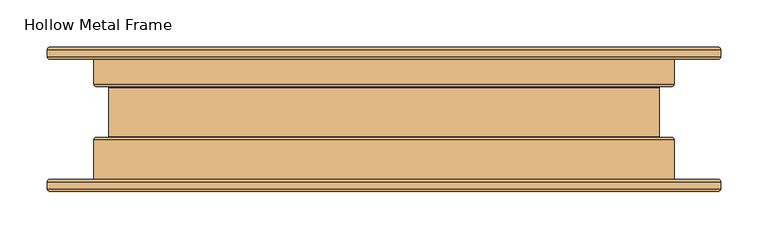
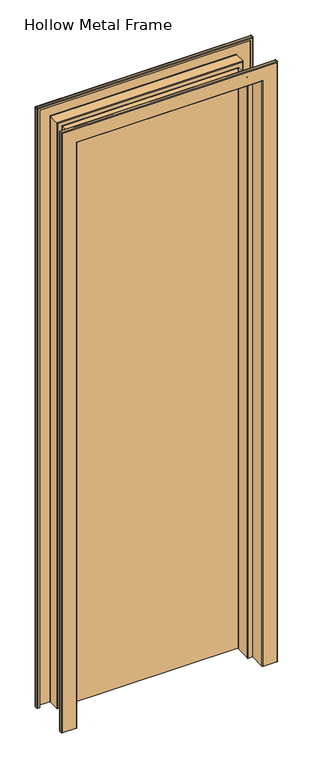
"""IFC4 building model written with IfcOpenShell, lengths in millimetres: door geometry, Hollow Metal Frame."""

from ifc_helpers import new_model, si_unit, frame, origin, origin_with_axes, place, context, project, spatial, polyline, circle_curve, ellipse_curve, outline, extrude, source, transform, mapped, element, save
from ifc_brep_helpers import plane_surface, cylinder_surface, revolved_surface, advanced_brep


def hollow_metal_frame_92897bd9(model_context):
    return source(origin(), model_context, "Body", "SolidModel", [
        advanced_brep(
        [(-353.02825, -63.5635, 0.0), (-347.6625, -63.5635, 0.0), (-347.6625, -65.11925, 0.0), (-353.02825, -65.11925, 0.0), (-354.04425, -66.13525, 0.0), (-354.04425, -73.66, 0.0), (-353.02825, -74.676, 0.0), (-307.37175, -74.676, 0.0), (-306.35575, -73.66, 0.0), (-306.35575, -21.68525, 0.0), (-303.784, -19.1135, 0.0), (-291.49675, -19.1135, 0.0), (-290.48075, -18.0975, 0.0), (-290.48075, 33.6931, 0.0), (-291.49675, 34.7091, 0.0), (-303.784, 34.7091, 0.0), (-306.35575, 37.28085, 0.0), (-306.35575, 73.5965, 0.0), (-307.37175, 74.6125, 0.0), (-353.02825, 74.6125, 0.0), (-354.04425, 73.5965, 0.0), (-354.04425, 66.07175, 0.0), (-353.02825, 65.05575, 0.0), (-347.6625, 65.05575, 0.0), (-347.6625, 63.5, 0.0), (-353.02825, 63.5, 0.0), (-355.6, 66.07175, 0.0), (-355.6, 73.5965, 0.0), (-353.02825, 76.16825, 0.0), (-307.37175, 76.16825, 0.0), (-304.8, 73.5965, 0.0), (-304.8, 37.28085, 0.0), (-303.784, 36.26485, 0.0), (-291.49675, 36.26485, 0.0), (-288.925, 33.6931, 0.0), (-288.925, -18.0975, 0.0), (-291.49675, -20.66925, 0.0), (-303.784, -20.66925, 0.0), (-304.8, -21.68525, 0.0), (-304.8, -73.66, 0.0), (-307.37175, -76.23175, 0.0), (-353.02825, -76.23175, 0.0), (-355.6, -73.66, 0.0), (-355.6, -66.13525, 0.0), (-355.6, -66.13525, 2082.8000001), (-353.02825, -63.5635, 2080.2282501), (-355.6, -73.66, 2082.8000001), (-353.02825, -76.23175, 2080.2282501), (-307.37175, -76.23175, 2034.5717501), (307.37175, -76.23175, 2034.5717501), (307.37175, -76.23175, 0.0), (353.02825, -76.23175, 0.0), (353.02825, -76.23175, 2080.2282501), (-304.8, -73.66, 2032.0000001), (-304.8, -21.68525, 2032.0000001), (-303.784, -20.66925, 2030.9840001), (-291.49675, -20.66925, 2018.6967501), (291.49675, -20.66925, 2018.6967501), (291.49675, -20.66925, 0.0), (303.784, -20.66925, 0.0), (303.784, -20.66925, 2030.9840001), (-288.925, -18.0975, 2016.1250001), (-288.925, 33.6931, 2016.1250001), (-291.49675, 36.26485, 2018.6967501), (-303.784, 36.26485, 2030.9840001), (303.784, 36.26485, 2030.9840001), (303.784, 36.26485, 0.0), (291.49675, 36.26485, 0.0), (291.49675, 36.26485, 2018.6967501), (-304.8, 37.28085, 2032.0000001), (-304.8, 73.5965, 2032.0000001), (-307.37175, 76.16825, 2034.5717501), (-353.02825, 76.16825, 2080.2282501), (353.02825, 76.16825, 2080.2282501), (353.02825, 76.16825, 0.0), (307.37175, 76.16825, 0.0), (307.37175, 76.16825, 2034.5717501), (-355.6, 73.5965, 2082.8000001), (-355.6, 66.07175, 2082.8000001), (-353.02825, 63.5, 2080.2282501), (-347.6625, 63.5, 2074.8625001), (347.6625, 63.5, 2074.8625001), (347.6625, 63.5, 0.0), (353.02825, 63.5, 0.0), (353.02825, 63.5, 2080.2282501), (-347.6625, 65.05575, 2074.8625001), (-353.02825, 65.05575, 2080.2282501), (353.02825, 65.05575, 2080.2282501), (353.02825, 65.05575, 0.0), (347.6625, 65.05575, 0.0), (347.6625, 65.05575, 2074.8625001), (-354.04425, 66.07175, 2081.2442501), (-354.04425, 73.5965, 2081.2442501), (-353.02825, 74.6125, 2080.2282501), (-307.37175, 74.6125, 2034.5717501), (307.37175, 74.6125, 2034.5717501), (307.37175, 74.6125, 0.0), (353.02825, 74.6125, 0.0), (353.02825, 74.6125, 2080.2282501), (-306.35575, 73.5965, 2033.5557501), (-306.35575, 37.28085, 2033.5557501), (-303.784, 34.7091, 2030.9840001), (-291.49675, 34.7091, 2018.6967501), (291.49675, 34.7091, 2018.6967501), (291.49675, 34.7091, 0.0), (303.784, 34.7091, 0.0), (303.784, 34.7091, 2030.9840001), (-290.48075, 33.6931, 2017.6807501), (-290.48075, -18.0975, 2017.6807501), (-291.49675, -19.1135, 2018.6967501), (-303.784, -19.1135, 2030.9840001), (303.784, -19.1135, 2030.9840001), (303.784, -19.1135, 0.0), (291.49675, -19.1135, 0.0), (291.49675, -19.1135, 2018.6967501), (-306.35575, -21.68525, 2033.5557501), (-306.35575, -73.66, 2033.5557501), (-307.37175, -74.676, 2034.5717501), (-353.02825, -74.676, 2080.2282501), (353.02825, -74.676, 2080.2282501), (353.02825, -74.676, 0.0), (307.37175, -74.676, 0.0), (307.37175, -74.676, 2034.5717501), (-354.04425, -73.66, 2081.2442501), (-354.04425, -66.13525, 2081.2442501), (-353.02825, -65.11925, 2080.2282501), (-347.6625, -65.11925, 2074.8625001), (347.6625, -65.11925, 2074.8625001), (347.6625, -65.11925, 0.0), (353.02825, -65.11925, 0.0), (353.02825, -65.11925, 2080.2282501), (-347.6625, -63.5635, 2074.8625001), (353.02825, -63.5635, 2080.2282501), (353.02825, -63.5635, 0.0), (347.6625, -63.5635, 0.0), (347.6625, -63.5635, 2074.8625001), (355.6, -66.13525, 2082.8000001), (355.6, -73.66, 2082.8000001), (304.8, -73.66, 2032.0000001), (304.8, -21.68525, 2032.0000001), (288.925, -18.0975, 2016.1250001), (288.925, 33.6931, 2016.1250001), (304.8, 37.28085, 2032.0000001), (304.8, 73.5965, 2032.0000001), (355.6, 73.5965, 2082.8000001), (355.6, 66.07175, 2082.8000001), (354.04425, 66.07175, 2081.2442501), (354.04425, 73.5965, 2081.2442501), (306.35575, 73.5965, 2033.5557501), (306.35575, 37.28085, 2033.5557501), (290.48075, 33.6931, 2017.6807501), (290.48075, -18.0975, 2017.6807501), (306.35575, -21.68525, 2033.5557501), (306.35575, -73.66, 2033.5557501), (354.04425, -73.66, 2081.2442501), (354.04425, -66.13525, 2081.2442501), (355.6, -66.13525, 0.0), (355.6, -73.66, 0.0), (304.8, -73.66, 0.0), (304.8, -21.68525, 0.0), (288.925, -18.0975, 0.0), (288.925, 33.6931, 0.0), (304.8, 37.28085, 0.0), (304.8, 73.5965, 0.0), (355.6, 73.5965, 0.0), (355.6, 66.07175, 0.0), (354.04425, 66.07175, 0.0), (354.04425, 73.5965, 0.0), (306.35575, 73.5965, 0.0), (306.35575, 37.28085, 0.0), (290.48075, 33.6931, 0.0), (290.48075, -18.0975, 0.0), (306.35575, -21.68525, 0.0), (306.35575, -73.66, 0.0), (354.04425, -73.66, 0.0), (354.04425, -66.13525, 0.0)],
        [
            (0, 1),
            (1, 2),
            (2, 3),
            (3, 4, circle_curve(frame((-353.02825, -66.13525, 0.0), z_axis=(0.0, 0.0, 1.0), x_axis=(0.0, 1.0, 0.0)), 1.016)),
            (4, 5),
            (5, 6, circle_curve(frame((-353.02825, -73.66, 0.0), z_axis=(0.0, 0.0, 1.0), x_axis=(0.0, 1.0, 0.0)), 1.016)),
            (6, 7),
            (7, 8, circle_curve(frame((-307.37175, -73.66, 0.0), z_axis=(0.0, 0.0, 1.0), x_axis=(0.0, 1.0, 0.0)), 1.016)),
            (8, 9),
            (9, 10, circle_curve(frame((-303.784, -21.68525, 0.0), z_axis=(0.0, 0.0, -1.0), x_axis=(0.0, 1.0, 0.0)), 2.57175)),
            (10, 11),
            (11, 12, circle_curve(frame((-291.49675, -18.0975, 0.0), z_axis=(0.0, 0.0, 1.0), x_axis=(0.0, 1.0, 0.0)), 1.016)),
            (12, 13),
            (13, 14, circle_curve(frame((-291.49675, 33.6931, 0.0), z_axis=(0.0, 0.0, 1.0), x_axis=(0.0, 1.0, 0.0)), 1.016)),
            (14, 15),
            (15, 16, circle_curve(frame((-303.784, 37.28085, 0.0), z_axis=(0.0, 0.0, -1.0), x_axis=(0.0, 1.0, 0.0)), 2.57175)),
            (16, 17),
            (17, 18, circle_curve(frame((-307.37175, 73.5965, 0.0), z_axis=(0.0, 0.0, 1.0), x_axis=(0.0, 1.0, 0.0)), 1.016)),
            (18, 19),
            (19, 20, circle_curve(frame((-353.02825, 73.5965, 0.0), z_axis=(0.0, 0.0, 1.0), x_axis=(0.0, 1.0, 0.0)), 1.016)),
            (20, 21),
            (21, 22, circle_curve(frame((-353.02825, 66.07175, 0.0), z_axis=(0.0, 0.0, 1.0), x_axis=(0.0, 1.0, 0.0)), 1.016)),
            (22, 23),
            (23, 24),
            (24, 25),
            (25, 26, circle_curve(frame((-353.02825, 66.07175, 0.0), z_axis=(0.0, 0.0, -1.0), x_axis=(0.0, 1.0, 0.0)), 2.57175)),
            (26, 27),
            (27, 28, circle_curve(frame((-353.02825, 73.5965, 0.0), z_axis=(0.0, 0.0, -1.0), x_axis=(0.0, 1.0, 0.0)), 2.57175)),
            (28, 29),
            (29, 30, circle_curve(frame((-307.37175, 73.5965, 0.0), z_axis=(0.0, 0.0, -1.0), x_axis=(0.0, 1.0, 0.0)), 2.57175)),
            (30, 31),
            (31, 32, circle_curve(frame((-303.784, 37.28085, 0.0), z_axis=(0.0, 0.0, 1.0), x_axis=(0.0, 1.0, 0.0)), 1.016)),
            (32, 33),
            (33, 34, circle_curve(frame((-291.49675, 33.6931, 0.0), z_axis=(0.0, 0.0, -1.0), x_axis=(0.0, 1.0, 0.0)), 2.57175)),
            (34, 35),
            (35, 36, circle_curve(frame((-291.49675, -18.0975, 0.0), z_axis=(0.0, 0.0, -1.0), x_axis=(0.0, 1.0, 0.0)), 2.57175)),
            (36, 37),
            (37, 38, circle_curve(frame((-303.784, -21.68525, 0.0), z_axis=(0.0, 0.0, 1.0), x_axis=(0.0, 1.0, 0.0)), 1.016)),
            (38, 39),
            (39, 40, circle_curve(frame((-307.37175, -73.66, 0.0), z_axis=(0.0, 0.0, -1.0), x_axis=(0.0, 1.0, 0.0)), 2.57175)),
            (40, 41),
            (41, 42, circle_curve(frame((-353.02825, -73.66, 0.0), z_axis=(0.0, 0.0, -1.0), x_axis=(0.0, 1.0, 0.0)), 2.57175)),
            (42, 43),
            (43, 0, circle_curve(frame((-353.02825, -66.13525, 0.0), z_axis=(0.0, 0.0, -1.0), x_axis=(0.0, 1.0, 0.0)), 2.57175)),
            (43, 44),
            (44, 45, ellipse_curve(frame((-353.02825, -66.13525, 2080.2282501), z_axis=(-0.7071067811865475, 0.0, -0.7071067811865475), x_axis=(0.7071067811865474, 0.0, -0.7071067811865476)), 3.6370037, 2.57175)),
            (45, 0),
            (42, 46),
            (46, 44),
            (41, 47),
            (47, 46, ellipse_curve(frame((-353.02825, -73.66, 2080.2282501), z_axis=(-0.7071067811865475, 0.0, -0.7071067811865475), x_axis=(0.7071067811865474, 0.0, -0.7071067811865476)), 3.6370037, 2.57175)),
            (40, 48),
            (48, 49),
            (49, 50),
            (50, 51),
            (51, 52),
            (52, 47),
            (39, 53),
            (53, 48, ellipse_curve(frame((-307.37175, -73.66, 2034.5717501), z_axis=(-0.7071067811865475, 0.0, -0.7071067811865475), x_axis=(0.7071067811865474, 0.0, -0.7071067811865476)), 3.6370037, 2.57175)),
            (38, 54),
            (54, 53),
            (37, 55),
            (55, 54, ellipse_curve(frame((-303.784, -21.68525, 2030.9840001), z_axis=(0.7071067811865475, 0.0, 0.7071067811865475), x_axis=(-0.7071067811865474, 0.0, 0.7071067811865476)), 1.436841, 1.016)),
            (36, 56),
            (56, 57),
            (57, 58),
            (58, 59),
            (59, 60),
            (60, 55),
            (35, 61),
            (61, 56, ellipse_curve(frame((-291.49675, -18.0975, 2018.6967501), z_axis=(-0.7071067811865475, 0.0, -0.7071067811865475), x_axis=(0.7071067811865474, 0.0, -0.7071067811865476)), 3.6370037, 2.57175)),
            (34, 62),
            (62, 61),
            (33, 63),
            (63, 62, ellipse_curve(frame((-291.49675, 33.6931, 2018.6967501), z_axis=(-0.7071067811865475, 0.0, -0.7071067811865475), x_axis=(0.7071067811865474, 0.0, -0.7071067811865476)), 3.6370037, 2.57175)),
            (32, 64),
            (64, 65),
            (65, 66),
            (66, 67),
            (67, 68),
            (68, 63),
            (31, 69),
            (69, 64, ellipse_curve(frame((-303.784, 37.28085, 2030.9840001), z_axis=(0.7071067811865475, 0.0, 0.7071067811865475), x_axis=(-0.7071067811865474, 0.0, 0.7071067811865476)), 1.436841, 1.016)),
            (30, 70),
            (70, 69),
            (29, 71),
            (71, 70, ellipse_curve(frame((-307.37175, 73.5965, 2034.5717501), z_axis=(-0.7071067811865475, 0.0, -0.7071067811865475), x_axis=(0.7071067811865474, 0.0, -0.7071067811865476)), 3.6370037, 2.57175)),
            (28, 72),
            (72, 73),
            (73, 74),
            (74, 75),
            (75, 76),
            (76, 71),
            (27, 77),
            (77, 72, ellipse_curve(frame((-353.02825, 73.5965, 2080.2282501), z_axis=(-0.7071067811865475, 0.0, -0.7071067811865475), x_axis=(0.7071067811865474, 0.0, -0.7071067811865476)), 3.6370037, 2.57175)),
            (26, 78),
            (78, 77),
            (25, 79),
            (79, 78, ellipse_curve(frame((-353.02825, 66.07175, 2080.2282501), z_axis=(-0.7071067811865475, 0.0, -0.7071067811865475), x_axis=(0.7071067811865474, 0.0, -0.7071067811865476)), 3.6370037, 2.57175)),
            (24, 80),
            (80, 81),
            (81, 82),
            (82, 83),
            (83, 84),
            (84, 79),
            (23, 85),
            (85, 80),
            (22, 86),
            (86, 87),
            (87, 88),
            (88, 89),
            (89, 90),
            (90, 85),
            (21, 91),
            (91, 86, ellipse_curve(frame((-353.02825, 66.07175, 2080.2282501), z_axis=(0.7071067811865475, 0.0, 0.7071067811865475), x_axis=(-0.7071067811865474, 0.0, 0.7071067811865476)), 1.436841, 1.016)),
            (20, 92),
            (92, 91),
            (19, 93),
            (93, 92, ellipse_curve(frame((-353.02825, 73.5965, 2080.2282501), z_axis=(0.7071067811865475, 0.0, 0.7071067811865475), x_axis=(-0.7071067811865474, 0.0, 0.7071067811865476)), 1.436841, 1.016)),
            (18, 94),
            (94, 95),
            (95, 96),
            (96, 97),
            (97, 98),
            (98, 93),
            (17, 99),
            (99, 94, ellipse_curve(frame((-307.37175, 73.5965, 2034.5717501), z_axis=(0.7071067811865475, 0.0, 0.7071067811865475), x_axis=(-0.7071067811865474, 0.0, 0.7071067811865476)), 1.436841, 1.016)),
            (16, 100),
            (100, 99),
            (15, 101),
            (101, 100, ellipse_curve(frame((-303.784, 37.28085, 2030.9840001), z_axis=(-0.7071067811865475, 0.0, -0.7071067811865475), x_axis=(0.7071067811865474, 0.0, -0.7071067811865476)), 3.6370037, 2.57175)),
            (14, 102),
            (102, 103),
            (103, 104),
            (104, 105),
            (105, 106),
            (106, 101),
            (13, 107),
            (107, 102, ellipse_curve(frame((-291.49675, 33.6931, 2018.6967501), z_axis=(0.7071067811865475, 0.0, 0.7071067811865475), x_axis=(-0.7071067811865474, 0.0, 0.7071067811865476)), 1.436841, 1.016)),
            (12, 108),
            (108, 107),
            (11, 109),
            (109, 108, ellipse_curve(frame((-291.49675, -18.0975, 2018.6967501), z_axis=(0.7071067811865475, 0.0, 0.7071067811865475), x_axis=(-0.7071067811865474, 0.0, 0.7071067811865476)), 1.436841, 1.016)),
            (10, 110),
            (110, 111),
            (111, 112),
            (112, 113),
            (113, 114),
            (114, 109),
            (9, 115),
            (115, 110, ellipse_curve(frame((-303.784, -21.68525, 2030.9840001), z_axis=(-0.7071067811865475, 0.0, -0.7071067811865475), x_axis=(0.7071067811865474, 0.0, -0.7071067811865476)), 3.6370037, 2.57175)),
            (8, 116),
            (116, 115),
            (7, 117),
            (117, 116, ellipse_curve(frame((-307.37175, -73.66, 2034.5717501), z_axis=(0.7071067811865475, 0.0, 0.7071067811865475), x_axis=(-0.7071067811865474, 0.0, 0.7071067811865476)), 1.436841, 1.016)),
            (6, 118),
            (118, 119),
            (119, 120),
            (120, 121),
            (121, 122),
            (122, 117),
            (5, 123),
            (123, 118, ellipse_curve(frame((-353.02825, -73.66, 2080.2282501), z_axis=(0.7071067811865475, 0.0, 0.7071067811865475), x_axis=(-0.7071067811865474, 0.0, 0.7071067811865476)), 1.436841, 1.016)),
            (4, 124),
            (124, 123),
            (3, 125),
            (125, 124, ellipse_curve(frame((-353.02825, -66.13525, 2080.2282501), z_axis=(0.7071067811865475, 0.0, 0.7071067811865475), x_axis=(-0.7071067811865474, 0.0, 0.7071067811865476)), 1.436841, 1.016)),
            (2, 126),
            (126, 127),
            (127, 128),
            (128, 129),
            (129, 130),
            (130, 125),
            (1, 131),
            (131, 126),
            (45, 132),
            (132, 133),
            (133, 134),
            (134, 135),
            (135, 131),
            (44, 136),
            (136, 132, ellipse_curve(frame((353.02825, -66.13525, 2080.2282501), z_axis=(-0.7071067811865475, 0.0, 0.7071067811865475), x_axis=(-0.7071067811865476, 0.0, -0.7071067811865474)), 3.6370037, 2.57175)),
            (46, 137),
            (137, 136),
            (52, 137, ellipse_curve(frame((353.02825, -73.66, 2080.2282501), z_axis=(-0.7071067811865475, 0.0, 0.7071067811865475), x_axis=(-0.7071067811865476, 0.0, -0.7071067811865474)), 3.6370037, 2.57175)),
            (53, 138),
            (138, 49, ellipse_curve(frame((307.37175, -73.66, 2034.5717501), z_axis=(-0.7071067811865475, 0.0, 0.7071067811865475), x_axis=(-0.7071067811865476, 0.0, -0.7071067811865474)), 3.6370037, 2.57175)),
            (54, 139),
            (139, 138),
            (60, 139, ellipse_curve(frame((303.784, -21.68525, 2030.9840001), z_axis=(0.7071067811865475, 0.0, -0.7071067811865475), x_axis=(0.7071067811865476, 0.0, 0.7071067811865474)), 1.436841, 1.016)),
            (61, 140),
            (140, 57, ellipse_curve(frame((291.49675, -18.0975, 2018.6967501), z_axis=(-0.7071067811865475, 0.0, 0.7071067811865475), x_axis=(-0.7071067811865476, 0.0, -0.7071067811865474)), 3.6370037, 2.57175)),
            (62, 141),
            (141, 140),
            (68, 141, ellipse_curve(frame((291.49675, 33.6931, 2018.6967501), z_axis=(-0.7071067811865475, 0.0, 0.7071067811865475), x_axis=(-0.7071067811865476, 0.0, -0.7071067811865474)), 3.6370037, 2.57175)),
            (69, 142),
            (142, 65, ellipse_curve(frame((303.784, 37.28085, 2030.9840001), z_axis=(0.7071067811865475, 0.0, -0.7071067811865475), x_axis=(0.7071067811865476, 0.0, 0.7071067811865474)), 1.436841, 1.016)),
            (70, 143),
            (143, 142),
            (76, 143, ellipse_curve(frame((307.37175, 73.5965, 2034.5717501), z_axis=(-0.7071067811865475, 0.0, 0.7071067811865475), x_axis=(-0.7071067811865476, 0.0, -0.7071067811865474)), 3.6370037, 2.57175)),
            (77, 144),
            (144, 73, ellipse_curve(frame((353.02825, 73.5965, 2080.2282501), z_axis=(-0.7071067811865475, 0.0, 0.7071067811865475), x_axis=(-0.7071067811865476, 0.0, -0.7071067811865474)), 3.6370037, 2.57175)),
            (78, 145),
            (145, 144),
            (84, 145, ellipse_curve(frame((353.02825, 66.07175, 2080.2282501), z_axis=(-0.7071067811865475, 0.0, 0.7071067811865475), x_axis=(-0.7071067811865476, 0.0, -0.7071067811865474)), 3.6370037, 2.57175)),
            (90, 81),
            (91, 146),
            (146, 87, ellipse_curve(frame((353.02825, 66.07175, 2080.2282501), z_axis=(0.7071067811865475, 0.0, -0.7071067811865475), x_axis=(0.7071067811865476, 0.0, 0.7071067811865474)), 1.436841, 1.016)),
            (92, 147),
            (147, 146),
            (98, 147, ellipse_curve(frame((353.02825, 73.5965, 2080.2282501), z_axis=(0.7071067811865475, 0.0, -0.7071067811865475), x_axis=(0.7071067811865476, 0.0, 0.7071067811865474)), 1.436841, 1.016)),
            (99, 148),
            (148, 95, ellipse_curve(frame((307.37175, 73.5965, 2034.5717501), z_axis=(0.7071067811865475, 0.0, -0.7071067811865475), x_axis=(0.7071067811865476, 0.0, 0.7071067811865474)), 1.436841, 1.016)),
            (100, 149),
            (149, 148),
            (106, 149, ellipse_curve(frame((303.784, 37.28085, 2030.9840001), z_axis=(-0.7071067811865475, 0.0, 0.7071067811865475), x_axis=(-0.7071067811865476, 0.0, -0.7071067811865474)), 3.6370037, 2.57175)),
            (107, 150),
            (150, 103, ellipse_curve(frame((291.49675, 33.6931, 2018.6967501), z_axis=(0.7071067811865475, 0.0, -0.7071067811865475), x_axis=(0.7071067811865476, 0.0, 0.7071067811865474)), 1.436841, 1.016)),
            (108, 151),
            (151, 150),
            (114, 151, ellipse_curve(frame((291.49675, -18.0975, 2018.6967501), z_axis=(0.7071067811865475, 0.0, -0.7071067811865475), x_axis=(0.7071067811865476, 0.0, 0.7071067811865474)), 1.436841, 1.016)),
            (115, 152),
            (152, 111, ellipse_curve(frame((303.784, -21.68525, 2030.9840001), z_axis=(-0.7071067811865475, 0.0, 0.7071067811865475), x_axis=(-0.7071067811865476, 0.0, -0.7071067811865474)), 3.6370037, 2.57175)),
            (116, 153),
            (153, 152),
            (122, 153, ellipse_curve(frame((307.37175, -73.66, 2034.5717501), z_axis=(0.7071067811865475, 0.0, -0.7071067811865475), x_axis=(0.7071067811865476, 0.0, 0.7071067811865474)), 1.436841, 1.016)),
            (123, 154),
            (154, 119, ellipse_curve(frame((353.02825, -73.66, 2080.2282501), z_axis=(0.7071067811865475, 0.0, -0.7071067811865475), x_axis=(0.7071067811865476, 0.0, 0.7071067811865474)), 1.436841, 1.016)),
            (124, 155),
            (155, 154),
            (130, 155, ellipse_curve(frame((353.02825, -66.13525, 2080.2282501), z_axis=(0.7071067811865475, 0.0, -0.7071067811865475), x_axis=(0.7071067811865476, 0.0, 0.7071067811865474)), 1.436841, 1.016)),
            (135, 127),
            (133, 156, circle_curve(frame((353.02825, -66.13525, 0.0), z_axis=(0.0, 0.0, -1.0), x_axis=(0.0, 1.0, 0.0)), 2.57175)),
            (156, 157),
            (157, 51, circle_curve(frame((353.02825, -73.66, 0.0), z_axis=(0.0, 0.0, -1.0), x_axis=(0.0, 1.0, 0.0)), 2.57175)),
            (50, 158, circle_curve(frame((307.37175, -73.66, 0.0), z_axis=(0.0, 0.0, -1.0), x_axis=(0.0, 1.0, 0.0)), 2.57175)),
            (158, 159),
            (159, 59, circle_curve(frame((303.784, -21.68525, 0.0), z_axis=(0.0, 0.0, 1.0), x_axis=(0.0, 1.0, 0.0)), 1.016)),
            (58, 160, circle_curve(frame((291.49675, -18.0975, 0.0), z_axis=(0.0, 0.0, -1.0), x_axis=(0.0, 1.0, 0.0)), 2.57175)),
            (160, 161),
            (161, 67, circle_curve(frame((291.49675, 33.6931, 0.0), z_axis=(0.0, 0.0, -1.0), x_axis=(0.0, 1.0, 0.0)), 2.57175)),
            (66, 162, circle_curve(frame((303.784, 37.28085, 0.0), z_axis=(0.0, 0.0, 1.0), x_axis=(0.0, 1.0, 0.0)), 1.016)),
            (162, 163),
            (163, 75, circle_curve(frame((307.37175, 73.5965, 0.0), z_axis=(0.0, 0.0, -1.0), x_axis=(0.0, 1.0, 0.0)), 2.57175)),
            (74, 164, circle_curve(frame((353.02825, 73.5965, 0.0), z_axis=(0.0, 0.0, -1.0), x_axis=(0.0, 1.0, 0.0)), 2.57175)),
            (164, 165),
            (165, 83, circle_curve(frame((353.02825, 66.07175, 0.0), z_axis=(0.0, 0.0, -1.0), x_axis=(0.0, 1.0, 0.0)), 2.57175)),
            (82, 89),
            (88, 166, circle_curve(frame((353.02825, 66.07175, 0.0), z_axis=(0.0, 0.0, 1.0), x_axis=(0.0, 1.0, 0.0)), 1.016)),
            (166, 167),
            (167, 97, circle_curve(frame((353.02825, 73.5965, 0.0), z_axis=(0.0, 0.0, 1.0), x_axis=(0.0, 1.0, 0.0)), 1.016)),
            (96, 168, circle_curve(frame((307.37175, 73.5965, 0.0), z_axis=(0.0, 0.0, 1.0), x_axis=(0.0, 1.0, 0.0)), 1.016)),
            (168, 169),
            (169, 105, circle_curve(frame((303.784, 37.28085, 0.0), z_axis=(0.0, 0.0, -1.0), x_axis=(0.0, 1.0, 0.0)), 2.57175)),
            (104, 170, circle_curve(frame((291.49675, 33.6931, 0.0), z_axis=(0.0, 0.0, 1.0), x_axis=(0.0, 1.0, 0.0)), 1.016)),
            (170, 171),
            (171, 113, circle_curve(frame((291.49675, -18.0975, 0.0), z_axis=(0.0, 0.0, 1.0), x_axis=(0.0, 1.0, 0.0)), 1.016)),
            (112, 172, circle_curve(frame((303.784, -21.68525, 0.0), z_axis=(0.0, 0.0, -1.0), x_axis=(0.0, 1.0, 0.0)), 2.57175)),
            (172, 173),
            (173, 121, circle_curve(frame((307.37175, -73.66, 0.0), z_axis=(0.0, 0.0, 1.0), x_axis=(0.0, 1.0, 0.0)), 1.016)),
            (120, 174, circle_curve(frame((353.02825, -73.66, 0.0), z_axis=(0.0, 0.0, 1.0), x_axis=(0.0, 1.0, 0.0)), 1.016)),
            (174, 175),
            (175, 129, circle_curve(frame((353.02825, -66.13525, 0.0), z_axis=(0.0, 0.0, 1.0), x_axis=(0.0, 1.0, 0.0)), 1.016)),
            (128, 134),
            (136, 156),
            (137, 157),
            (138, 158),
            (139, 159),
            (140, 160),
            (141, 161),
            (142, 162),
            (143, 163),
            (144, 164),
            (145, 165),
            (146, 166),
            (147, 167),
            (148, 168),
            (149, 169),
            (150, 170),
            (151, 171),
            (152, 172),
            (153, 173),
            (154, 174),
            (155, 175),
        ],
        [
            plane_surface(frame((-315.9125, 63.5, 0.0), z_axis=(0.0, 0.0, -1.0), x_axis=(1.0, 0.0, 0.0))),
            cylinder_surface(frame((-353.02825, -66.13525, 0.0), z_axis=(0.0, 0.0, -1.0), x_axis=(0.0, 1.0, 0.0)), 2.57175),
            plane_surface(frame((-355.6, -66.13525, 0.0), z_axis=(-1.0, 0.0, 0.0), x_axis=(0.0, 0.0, 1.0))),
            cylinder_surface(frame((-353.02825, -73.66, 0.0), z_axis=(0.0, 0.0, -1.0), x_axis=(0.0, 1.0, 0.0)), 2.57175),
            plane_surface(frame((-353.02825, -76.23175, 0.0), z_axis=(0.0, -1.0, 0.0), x_axis=(0.0, 0.0, 1.0))),
            cylinder_surface(frame((-307.37175, -73.66, 0.0), z_axis=(0.0, 0.0, -1.0), x_axis=(0.0, 1.0, 0.0)), 2.57175),
            plane_surface(frame((-304.8, -73.66, 0.0), z_axis=(1.0, 0.0, 0.0), x_axis=(0.0, 0.0, 1.0))),
            revolved_surface(polyline([(-303.784, -20.669249999999998, 2032.0000001145868), (-303.784, -20.669249999999998, 0.0)]), (-303.784, -21.68525, 0.0), (0.0, 0.0, 1.0)),
            plane_surface(frame((-303.784, -20.66925, 0.0), z_axis=(0.0, -1.0, 0.0), x_axis=(0.0, 0.0, 1.0))),
            cylinder_surface(frame((-291.49675, -18.0975, 0.0), z_axis=(0.0, 0.0, -1.0), x_axis=(0.0, 1.0, 0.0)), 2.57175),
            plane_surface(frame((-288.925, -18.0975, 0.0), z_axis=(1.0, 0.0, 0.0), x_axis=(0.0, 0.0, 1.0))),
            cylinder_surface(frame((-291.49675, 33.6931, 0.0), z_axis=(0.0, 0.0, -1.0), x_axis=(0.0, 1.0, 0.0)), 2.57175),
            plane_surface(frame((-291.49675, 36.26485, 0.0), z_axis=(0.0, 1.0, 0.0), x_axis=(0.0, 0.0, 1.0))),
            revolved_surface(polyline([(-303.784, 38.29685, 2032.0000001145868), (-303.784, 38.29685, 0.0)]), (-303.784, 37.28085, 0.0), (0.0, 0.0, 1.0)),
            plane_surface(frame((-304.8, 37.28085, 0.0), z_axis=(1.0, 0.0, 0.0), x_axis=(0.0, 0.0, 1.0))),
            cylinder_surface(frame((-307.37175, 73.5965, 0.0), z_axis=(0.0, 0.0, -1.0), x_axis=(0.0, 1.0, 0.0)), 2.57175),
            plane_surface(frame((-307.37175, 76.16825, 0.0), z_axis=(0.0, 1.0, 0.0), x_axis=(0.0, 0.0, 1.0))),
            cylinder_surface(frame((-353.02825, 73.5965, 0.0), z_axis=(0.0, 0.0, -1.0), x_axis=(0.0, 1.0, 0.0)), 2.57175),
            plane_surface(frame((-355.6, 73.5965, 0.0), z_axis=(-1.0, 0.0, 0.0), x_axis=(0.0, 0.0, 1.0))),
            cylinder_surface(frame((-353.02825, 66.07175, 0.0), z_axis=(0.0, 0.0, -1.0), x_axis=(0.0, 1.0, 0.0)), 2.57175),
            plane_surface(frame((-353.02825, 63.5, 0.0), z_axis=(0.0, -1.0, 0.0), x_axis=(0.0, 0.0, 1.0))),
            plane_surface(frame((-347.6625, 63.5, 0.0), z_axis=(1.0, 0.0, 0.0), x_axis=(0.0, 0.0, 1.0))),
            plane_surface(frame((-347.6625, 65.05575, 0.0), z_axis=(0.0, 1.0, 0.0), x_axis=(0.0, 0.0, 1.0))),
            revolved_surface(polyline([(-353.02825, 67.08775, 2081.244250114587), (-353.02825, 67.08775, 0.0)]), (-353.02825, 66.07175, 0.0), (0.0, 0.0, 1.0)),
            plane_surface(frame((-354.04425, 66.07175, 0.0), z_axis=(1.0, 0.0, 0.0), x_axis=(0.0, 0.0, 1.0))),
            revolved_surface(polyline([(-353.02825, 74.61250000000001, 2081.244250114587), (-353.02825, 74.61250000000001, 0.0)]), (-353.02825, 73.5965, 0.0), (0.0, 0.0, 1.0)),
            plane_surface(frame((-353.02825, 74.6125, 0.0), z_axis=(0.0, -1.0, 0.0), x_axis=(0.0, 0.0, 1.0))),
            revolved_surface(polyline([(-307.37175, 74.61250000000001, 2035.5877501145867), (-307.37175, 74.61250000000001, 0.0)]), (-307.37175, 73.5965, 0.0), (0.0, 0.0, 1.0)),
            plane_surface(frame((-306.35575, 73.5965, 0.0), z_axis=(-1.0, 0.0, 0.0), x_axis=(0.0, 0.0, 1.0))),
            cylinder_surface(frame((-303.784, 37.28085, 0.0), z_axis=(0.0, 0.0, -1.0), x_axis=(0.0, 1.0, 0.0)), 2.57175),
            plane_surface(frame((-303.784, 34.7091, 0.0), z_axis=(0.0, -1.0, 0.0), x_axis=(0.0, 0.0, 1.0))),
            revolved_surface(polyline([(-291.49675, 34.7091, 2019.7127501145867), (-291.49675, 34.7091, 0.0)]), (-291.49675, 33.6931, 0.0), (0.0, 0.0, 1.0)),
            plane_surface(frame((-290.48075, 33.6931, 0.0), z_axis=(-1.0, 0.0, 0.0), x_axis=(0.0, 0.0, 1.0))),
            revolved_surface(polyline([(-291.49675, -17.0815, 2019.7127501145867), (-291.49675, -17.0815, 0.0)]), (-291.49675, -18.0975, 0.0), (0.0, 0.0, 1.0)),
            plane_surface(frame((-291.49675, -19.1135, 0.0), z_axis=(0.0, 1.0, 0.0), x_axis=(0.0, 0.0, 1.0))),
            cylinder_surface(frame((-303.784, -21.68525, 0.0), z_axis=(0.0, 0.0, -1.0), x_axis=(0.0, 1.0, 0.0)), 2.57175),
            plane_surface(frame((-306.35575, -21.68525, 0.0), z_axis=(-1.0, 0.0, 0.0), x_axis=(0.0, 0.0, 1.0))),
            revolved_surface(polyline([(-307.37175, -72.64399999999999, 2035.5877501145867), (-307.37175, -72.64399999999999, 0.0)]), (-307.37175, -73.66, 0.0), (0.0, 0.0, 1.0)),
            plane_surface(frame((-307.37175, -74.676, 0.0), z_axis=(0.0, 1.0, 0.0), x_axis=(0.0, 0.0, 1.0))),
            revolved_surface(polyline([(-353.02825, -72.64399999999999, 2081.244250114587), (-353.02825, -72.64399999999999, 0.0)]), (-353.02825, -73.66, 0.0), (0.0, 0.0, 1.0)),
            plane_surface(frame((-354.04425, -73.66, 0.0), z_axis=(1.0, 0.0, 0.0), x_axis=(0.0, 0.0, 1.0))),
            revolved_surface(polyline([(-353.02825, -65.11925, 2081.244250114587), (-353.02825, -65.11925, 0.0)]), (-353.02825, -66.13525, 0.0), (0.0, 0.0, 1.0)),
            plane_surface(frame((-353.02825, -65.11925, 0.0), z_axis=(0.0, -1.0, 0.0), x_axis=(0.0, 0.0, 1.0))),
            plane_surface(frame((-347.6625, -65.11925, 0.0), z_axis=(1.0, 0.0, 0.0), x_axis=(0.0, 0.0, 1.0))),
            plane_surface(frame((-347.6625, -63.5635, 0.0), z_axis=(0.0, 1.0, 0.0), x_axis=(0.0, 0.0, 1.0))),
            cylinder_surface(frame((-315.9125, -66.13525, 2080.2282501), z_axis=(-1.0, 0.0, 0.0), x_axis=(0.0, 1.0, 0.0)), 2.57175),
            plane_surface(frame((-355.6, -66.13525, 2082.8000001), z_axis=(0.0, 0.0, 1.0), x_axis=(1.0, 0.0, 0.0))),
            cylinder_surface(frame((-315.9125, -73.66, 2080.2282501), z_axis=(-1.0, 0.0, 0.0), x_axis=(0.0, 1.0, 0.0)), 2.57175),
            cylinder_surface(frame((-315.9125, -73.66, 2034.5717501), z_axis=(-1.0, 0.0, 0.0), x_axis=(0.0, 1.0, 0.0)), 2.57175),
            plane_surface(frame((-304.8, -73.66, 2032.0000001), z_axis=(0.0, 0.0, -1.0), x_axis=(1.0, 0.0, 0.0))),
            revolved_surface(polyline([(304.8000000145869, -20.669249999999998, 2030.9840001), (-304.80000001458683, -20.669249999999998, 2030.9840001)]), (-315.9125, -21.68525, 2030.9840001), (1.0, 0.0, 0.0)),
            cylinder_surface(frame((-315.9125, -18.0975, 2018.6967501), z_axis=(-1.0, 0.0, 0.0), x_axis=(0.0, 1.0, 0.0)), 2.57175),
            plane_surface(frame((-288.925, -18.0975, 2016.1250001), z_axis=(0.0, 0.0, -1.0), x_axis=(1.0, 0.0, 0.0))),
            cylinder_surface(frame((-315.9125, 33.6931, 2018.6967501), z_axis=(-1.0, 0.0, 0.0), x_axis=(0.0, 1.0, 0.0)), 2.57175),
            revolved_surface(polyline([(304.8000000145869, 38.29685, 2030.9840001), (-304.80000001458683, 38.29685, 2030.9840001)]), (-315.9125, 37.28085, 2030.9840001), (1.0, 0.0, 0.0)),
            plane_surface(frame((-304.8, 37.28085, 2032.0000001), z_axis=(0.0, 0.0, -1.0), x_axis=(1.0, 0.0, 0.0))),
            cylinder_surface(frame((-315.9125, 73.5965, 2034.5717501), z_axis=(-1.0, 0.0, 0.0), x_axis=(0.0, 1.0, 0.0)), 2.57175),
            cylinder_surface(frame((-315.9125, 73.5965, 2080.2282501), z_axis=(-1.0, 0.0, 0.0), x_axis=(0.0, 1.0, 0.0)), 2.57175),
            plane_surface(frame((-355.6, 73.5965, 2082.8000001), z_axis=(0.0, 0.0, 1.0), x_axis=(1.0, 0.0, 0.0))),
            cylinder_surface(frame((-315.9125, 66.07175, 2080.2282501), z_axis=(-1.0, 0.0, 0.0), x_axis=(0.0, 1.0, 0.0)), 2.57175),
            plane_surface(frame((-347.6625, 63.5, 2074.8625001), z_axis=(0.0, 0.0, -1.0), x_axis=(1.0, 0.0, 0.0))),
            revolved_surface(polyline([(354.04425001458685, 67.08775, 2080.2282501), (-354.04425001458685, 67.08775, 2080.2282501)]), (-315.9125, 66.07175, 2080.2282501), (1.0, 0.0, 0.0)),
            plane_surface(frame((-354.04425, 66.07175, 2081.2442501), z_axis=(0.0, 0.0, -1.0), x_axis=(1.0, 0.0, 0.0))),
            revolved_surface(polyline([(354.04425001458685, 74.61250000000001, 2080.2282501), (-354.04425001458685, 74.61250000000001, 2080.2282501)]), (-315.9125, 73.5965, 2080.2282501), (1.0, 0.0, 0.0)),
            revolved_surface(polyline([(308.3877500145869, 74.61250000000001, 2034.5717501), (-308.38775001458686, 74.61250000000001, 2034.5717501)]), (-315.9125, 73.5965, 2034.5717501), (1.0, 0.0, 0.0)),
            plane_surface(frame((-306.35575, 73.5965, 2033.5557501), z_axis=(0.0, 0.0, 1.0), x_axis=(1.0, 0.0, 0.0))),
            cylinder_surface(frame((-315.9125, 37.28085, 2030.9840001), z_axis=(-1.0, 0.0, 0.0), x_axis=(0.0, 1.0, 0.0)), 2.57175),
            revolved_surface(polyline([(292.5127500145869, 34.7091, 2018.6967501), (-292.51275001458686, 34.7091, 2018.6967501)]), (-315.9125, 33.6931, 2018.6967501), (1.0, 0.0, 0.0)),
            plane_surface(frame((-290.48075, 33.6931, 2017.6807501), z_axis=(0.0, 0.0, 1.0), x_axis=(1.0, 0.0, 0.0))),
            revolved_surface(polyline([(292.5127500145869, -17.0815, 2018.6967501), (-292.51275001458686, -17.0815, 2018.6967501)]), (-315.9125, -18.0975, 2018.6967501), (1.0, 0.0, 0.0)),
            cylinder_surface(frame((-315.9125, -21.68525, 2030.9840001), z_axis=(-1.0, 0.0, 0.0), x_axis=(0.0, 1.0, 0.0)), 2.57175),
            plane_surface(frame((-306.35575, -21.68525, 2033.5557501), z_axis=(0.0, 0.0, 1.0), x_axis=(1.0, 0.0, 0.0))),
            revolved_surface(polyline([(308.3877500145869, -72.64399999999999, 2034.5717501), (-308.38775001458686, -72.64399999999999, 2034.5717501)]), (-315.9125, -73.66, 2034.5717501), (1.0, 0.0, 0.0)),
            revolved_surface(polyline([(354.04425001458685, -72.64399999999999, 2080.2282501), (-354.04425001458685, -72.64399999999999, 2080.2282501)]), (-315.9125, -73.66, 2080.2282501), (1.0, 0.0, 0.0)),
            plane_surface(frame((-354.04425, -73.66, 2081.2442501), z_axis=(0.0, 0.0, -1.0), x_axis=(1.0, 0.0, 0.0))),
            revolved_surface(polyline([(354.04425001458685, -65.11925, 2080.2282501), (-354.04425001458685, -65.11925, 2080.2282501)]), (-315.9125, -66.13525, 2080.2282501), (1.0, 0.0, 0.0)),
            plane_surface(frame((-347.6625, -65.11925, 2074.8625001), z_axis=(0.0, 0.0, -1.0), x_axis=(1.0, 0.0, 0.0))),
            plane_surface(frame((315.9125, 63.5, 0.0), z_axis=(0.0, 0.0, -1.0), x_axis=(-1.0, 0.0, 0.0))),
            cylinder_surface(frame((353.02825, -66.13525, 2043.1125001), z_axis=(0.0, 0.0, 1.0), x_axis=(0.0, 1.0, 0.0)), 2.57175),
            plane_surface(frame((355.6, -66.13525, 2082.8000001), z_axis=(1.0, 0.0, 0.0), x_axis=(0.0, 0.0, -1.0))),
            cylinder_surface(frame((353.02825, -73.66, 2043.1125001), z_axis=(0.0, 0.0, 1.0), x_axis=(0.0, 1.0, 0.0)), 2.57175),
            cylinder_surface(frame((307.37175, -73.66, 2043.1125001), z_axis=(0.0, 0.0, 1.0), x_axis=(0.0, 1.0, 0.0)), 2.57175),
            plane_surface(frame((304.8, -73.66, 2032.0000001), z_axis=(-1.0, 0.0, 0.0), x_axis=(0.0, 0.0, -1.0))),
            revolved_surface(polyline([(303.784, -20.669249999999998, 0.0), (303.784, -20.669249999999998, 2032.0000001145868)]), (303.784, -21.68525, 2043.1125001), (0.0, 0.0, -1.0)),
            cylinder_surface(frame((291.49675, -18.0975, 2043.1125001), z_axis=(0.0, 0.0, 1.0), x_axis=(0.0, 1.0, 0.0)), 2.57175),
            plane_surface(frame((288.925, -18.0975, 2016.1250001), z_axis=(-1.0, 0.0, 0.0), x_axis=(0.0, 0.0, -1.0))),
            cylinder_surface(frame((291.49675, 33.6931, 2043.1125001), z_axis=(0.0, 0.0, 1.0), x_axis=(0.0, 1.0, 0.0)), 2.57175),
            revolved_surface(polyline([(303.784, 38.29685, 0.0), (303.784, 38.29685, 2032.0000001145868)]), (303.784, 37.28085, 2043.1125001), (0.0, 0.0, -1.0)),
            plane_surface(frame((304.8, 37.28085, 2032.0000001), z_axis=(-1.0, 0.0, 0.0), x_axis=(0.0, 0.0, -1.0))),
            cylinder_surface(frame((307.37175, 73.5965, 2043.1125001), z_axis=(0.0, 0.0, 1.0), x_axis=(0.0, 1.0, 0.0)), 2.57175),
            cylinder_surface(frame((353.02825, 73.5965, 2043.1125001), z_axis=(0.0, 0.0, 1.0), x_axis=(0.0, 1.0, 0.0)), 2.57175),
            plane_surface(frame((355.6, 73.5965, 2082.8000001), z_axis=(1.0, 0.0, 0.0), x_axis=(0.0, 0.0, -1.0))),
            cylinder_surface(frame((353.02825, 66.07175, 2043.1125001), z_axis=(0.0, 0.0, 1.0), x_axis=(0.0, 1.0, 0.0)), 2.57175),
            plane_surface(frame((347.6625, 63.5, 2074.8625001), z_axis=(-1.0, 0.0, 0.0), x_axis=(0.0, 0.0, -1.0))),
            revolved_surface(polyline([(353.02825, 67.08775, 0.0), (353.02825, 67.08775, 2081.244250114587)]), (353.02825, 66.07175, 2043.1125001), (0.0, 0.0, -1.0)),
            plane_surface(frame((354.04425, 66.07175, 2081.2442501), z_axis=(-1.0, 0.0, 0.0), x_axis=(0.0, 0.0, -1.0))),
            revolved_surface(polyline([(353.02825, 74.61250000000001, 0.0), (353.02825, 74.61250000000001, 2081.244250114587)]), (353.02825, 73.5965, 2043.1125001), (0.0, 0.0, -1.0)),
            revolved_surface(polyline([(307.37175, 74.61250000000001, 0.0), (307.37175, 74.61250000000001, 2035.5877501145867)]), (307.37175, 73.5965, 2043.1125001), (0.0, 0.0, -1.0)),
            plane_surface(frame((306.35575, 73.5965, 2033.5557501), z_axis=(1.0, 0.0, 0.0), x_axis=(0.0, 0.0, -1.0))),
            cylinder_surface(frame((303.784, 37.28085, 2043.1125001), z_axis=(0.0, 0.0, 1.0), x_axis=(0.0, 1.0, 0.0)), 2.57175),
            revolved_surface(polyline([(291.49675, 34.7091, 0.0), (291.49675, 34.7091, 2019.7127501145867)]), (291.49675, 33.6931, 2043.1125001), (0.0, 0.0, -1.0)),
            plane_surface(frame((290.48075, 33.6931, 2017.6807501), z_axis=(1.0, 0.0, 0.0), x_axis=(0.0, 0.0, -1.0))),
            revolved_surface(polyline([(291.49675, -17.0815, 0.0), (291.49675, -17.0815, 2019.7127501145867)]), (291.49675, -18.0975, 2043.1125001), (0.0, 0.0, -1.0)),
            cylinder_surface(frame((303.784, -21.68525, 2043.1125001), z_axis=(0.0, 0.0, 1.0), x_axis=(0.0, 1.0, 0.0)), 2.57175),
            plane_surface(frame((306.35575, -21.68525, 2033.5557501), z_axis=(1.0, 0.0, 0.0), x_axis=(0.0, 0.0, -1.0))),
            revolved_surface(polyline([(307.37175, -72.64399999999999, 0.0), (307.37175, -72.64399999999999, 2035.5877501145867)]), (307.37175, -73.66, 2043.1125001), (0.0, 0.0, -1.0)),
            revolved_surface(polyline([(353.02825, -72.64399999999999, 0.0), (353.02825, -72.64399999999999, 2081.244250114587)]), (353.02825, -73.66, 2043.1125001), (0.0, 0.0, -1.0)),
            plane_surface(frame((354.04425, -73.66, 2081.2442501), z_axis=(-1.0, 0.0, 0.0), x_axis=(0.0, 0.0, -1.0))),
            revolved_surface(polyline([(353.02825, -65.11925, 0.0), (353.02825, -65.11925, 2081.244250114587)]), (353.02825, -66.13525, 2043.1125001), (0.0, 0.0, -1.0)),
            plane_surface(frame((347.6625, -65.11925, 2074.8625001), z_axis=(-1.0, 0.0, 0.0), x_axis=(0.0, 0.0, -1.0))),
        ],
        [
            (0, [[1, 2, 3, 4, 5, 6, 7, 8, 9, 10, 11, 12, 13, 14, 15, 16, 17, 18, 19, 20, 21, 22, 23, 24, 25, 26, 27, 28, 29, 30, 31, 32, 33, 34, 35, 36, 37, 38, 39, 40, 41, 42, 43, 44]]),
            (1, [[45, 46, 47, -44]]),
            (2, [[48, 49, -45, -43]]),
            (3, [[50, 51, -48, -42]]),
            (4, [[52, 53, 54, 55, 56, 57, -50, -41]]),
            (5, [[58, 59, -52, -40]]),
            (6, [[60, 61, -58, -39]]),
            (7, [[62, 63, -60, -38]]),
            (8, [[64, 65, 66, 67, 68, 69, -62, -37]]),
            (9, [[70, 71, -64, -36]]),
            (10, [[72, 73, -70, -35]]),
            (11, [[74, 75, -72, -34]]),
            (12, [[76, 77, 78, 79, 80, 81, -74, -33]]),
            (13, [[82, 83, -76, -32]]),
            (14, [[84, 85, -82, -31]]),
            (15, [[86, 87, -84, -30]]),
            (16, [[88, 89, 90, 91, 92, 93, -86, -29]]),
            (17, [[94, 95, -88, -28]]),
            (18, [[96, 97, -94, -27]]),
            (19, [[98, 99, -96, -26]]),
            (20, [[100, 101, 102, 103, 104, 105, -98, -25]]),
            (21, [[106, 107, -100, -24]]),
            (22, [[108, 109, 110, 111, 112, 113, -106, -23]]),
            (23, [[114, 115, -108, -22]]),
            (24, [[116, 117, -114, -21]]),
            (25, [[118, 119, -116, -20]]),
            (26, [[120, 121, 122, 123, 124, 125, -118, -19]]),
            (27, [[126, 127, -120, -18]]),
            (28, [[128, 129, -126, -17]]),
            (29, [[130, 131, -128, -16]]),
            (30, [[132, 133, 134, 135, 136, 137, -130, -15]]),
            (31, [[138, 139, -132, -14]]),
            (32, [[140, 141, -138, -13]]),
            (33, [[142, 143, -140, -12]]),
            (34, [[144, 145, 146, 147, 148, 149, -142, -11]]),
            (35, [[150, 151, -144, -10]]),
            (36, [[152, 153, -150, -9]]),
            (37, [[154, 155, -152, -8]]),
            (38, [[156, 157, 158, 159, 160, 161, -154, -7]]),
            (39, [[162, 163, -156, -6]]),
            (40, [[164, 165, -162, -5]]),
            (41, [[166, 167, -164, -4]]),
            (42, [[168, 169, 170, 171, 172, 173, -166, -3]]),
            (43, [[174, 175, -168, -2]]),
            (44, [[-47, 176, 177, 178, 179, 180, -174, -1]]),
            (45, [[181, 182, -176, -46]]),
            (46, [[183, 184, -181, -49]]),
            (47, [[-57, 185, -183, -51]]),
            (48, [[186, 187, -53, -59]]),
            (49, [[188, 189, -186, -61]]),
            (50, [[-69, 190, -188, -63]]),
            (51, [[191, 192, -65, -71]]),
            (52, [[193, 194, -191, -73]]),
            (53, [[-81, 195, -193, -75]]),
            (54, [[196, 197, -77, -83]]),
            (55, [[198, 199, -196, -85]]),
            (56, [[-93, 200, -198, -87]]),
            (57, [[201, 202, -89, -95]]),
            (58, [[203, 204, -201, -97]]),
            (59, [[-105, 205, -203, -99]]),
            (60, [[-113, 206, -101, -107]]),
            (61, [[207, 208, -109, -115]]),
            (62, [[209, 210, -207, -117]]),
            (63, [[-125, 211, -209, -119]]),
            (64, [[212, 213, -121, -127]]),
            (65, [[214, 215, -212, -129]]),
            (66, [[-137, 216, -214, -131]]),
            (67, [[217, 218, -133, -139]]),
            (68, [[219, 220, -217, -141]]),
            (69, [[-149, 221, -219, -143]]),
            (70, [[222, 223, -145, -151]]),
            (71, [[224, 225, -222, -153]]),
            (72, [[-161, 226, -224, -155]]),
            (73, [[227, 228, -157, -163]]),
            (74, [[229, 230, -227, -165]]),
            (75, [[-173, 231, -229, -167]]),
            (76, [[-180, 232, -169, -175]]),
            (77, [[233, 234, 235, -55, 236, 237, 238, -67, 239, 240, 241, -79, 242, 243, 244, -91, 245, 246, 247, -103, 248, -111, 249, 250, 251, -123, 252, 253, 254, -135, 255, 256, 257, -147, 258, 259, 260, -159, 261, 262, 263, -171, 264, -178]]),
            (78, [[265, -233, -177, -182]]),
            (79, [[266, -234, -265, -184]]),
            (80, [[-56, -235, -266, -185]]),
            (81, [[267, -236, -54, -187]]),
            (82, [[268, -237, -267, -189]]),
            (83, [[-68, -238, -268, -190]]),
            (84, [[269, -239, -66, -192]]),
            (85, [[270, -240, -269, -194]]),
            (86, [[-80, -241, -270, -195]]),
            (87, [[271, -242, -78, -197]]),
            (88, [[272, -243, -271, -199]]),
            (89, [[-92, -244, -272, -200]]),
            (90, [[273, -245, -90, -202]]),
            (91, [[274, -246, -273, -204]]),
            (92, [[-104, -247, -274, -205]]),
            (93, [[-112, -248, -102, -206]]),
            (94, [[275, -249, -110, -208]]),
            (95, [[276, -250, -275, -210]]),
            (96, [[-124, -251, -276, -211]]),
            (97, [[277, -252, -122, -213]]),
            (98, [[278, -253, -277, -215]]),
            (99, [[-136, -254, -278, -216]]),
            (100, [[279, -255, -134, -218]]),
            (101, [[280, -256, -279, -220]]),
            (102, [[-148, -257, -280, -221]]),
            (103, [[281, -258, -146, -223]]),
            (104, [[282, -259, -281, -225]]),
            (105, [[-160, -260, -282, -226]]),
            (106, [[283, -261, -158, -228]]),
            (107, [[284, -262, -283, -230]]),
            (108, [[-172, -263, -284, -231]]),
            (109, [[-179, -264, -170, -232]]),
        ],
    ),
        extrude(outline(polyline([(303.24425, 37.28085), (-303.24425, 37.28085), (-303.24425, 63.5), (303.24425, 63.5), (303.24425, 37.28085)])), origin_with_axes(), (0.0, 0.0, 1.0), 2032.0000001),
    ])


if __name__ == "__main__":
    model = new_model("IFC4")
    model_context = context("Model", 3, world=origin())
    ifc_project = project(units=[si_unit("LENGTHUNIT", "METRE", prefix="MILLI")], contexts=[model_context])
    site = spatial("IfcSite", under=ifc_project)
    building = spatial("IfcBuilding", under=site)
    placement = place(None, origin())
    hollow_metal_frame_shape = hollow_metal_frame_92897bd9(model_context)
    element("IfcDoor", 1, ObjectType="Hollow Metal Frame : 2' 0\"W x 6'-8\"H", at=placement, inside=building, context=model_context, shape_type="MappedRepresentation", body=[
        mapped(hollow_metal_frame_shape, transform((0.0, 0.0, 0.0), x_axis=(1.0, 0.0, 0.0), y_axis=(0.0, 1.0, 0.0), z_axis=(0.0, 0.0, 1.0))),
    ])
    save(model, "model.ifc")

# Revit data of these elements
# Type "Hollow Metal Frame : 2' 0\"W x 6'-8\"H"
#   Type Mark = "l"
#   Product Page URL = ""
#   Product Name = ""
#   Product Documentation Link = ""
#   Material = ""
#   DS_Hardware_Set_(SFT) = ""
#   DS_Frame_Type_(SFT) = ""
#   DS_Fire_Rating_(SFT) = ""
#   DS_Door_Type_(SFT) = ""
#   Analytic Construction = "<None>"
#   Frame Projection Ext. = 0' - 1"
#   Frame Projection Int. = 0' - 1"
#   Frame Width = 0' - 3"
#   Height = 6' - 8"
#   Width = 2' - 0"
#   Non-Kerfed = yes
#   Kerfed = no
#   Hollow Metal Casing = Metal-Dunbarton_Doors-White
#   Flush Door = Metal-Dunbarton_Doors-Aluminum
#   DS_Frame_Material_(SFT) = none
#   DS_Door_Material_(SFT) = none
#   URL = ""
#   Model = ""
#   Manufacturer = ""
#   Function = (empty or 0)
#   Wall Closure = (empty or 0)
#   Description = (empty or 0)
# Element 1 (IfcDoor, "Hollow Metal Frame : 2' 0\"W x 6'-8\"H")
#   Materials on its faces: "Metal-Dunbarton_Doors-White", "Metal-Dunbarton_Doors-Aluminum"
# Materials
#   "Metal-Dunbarton_Doors-White": class "Miscellaneous", colour RGB 230 233 236, transparency 0
#   "Metal-Dunbarton_Doors-Aluminum": class "System", colour RGB 143 142 141, transparency 0
